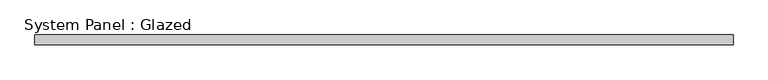
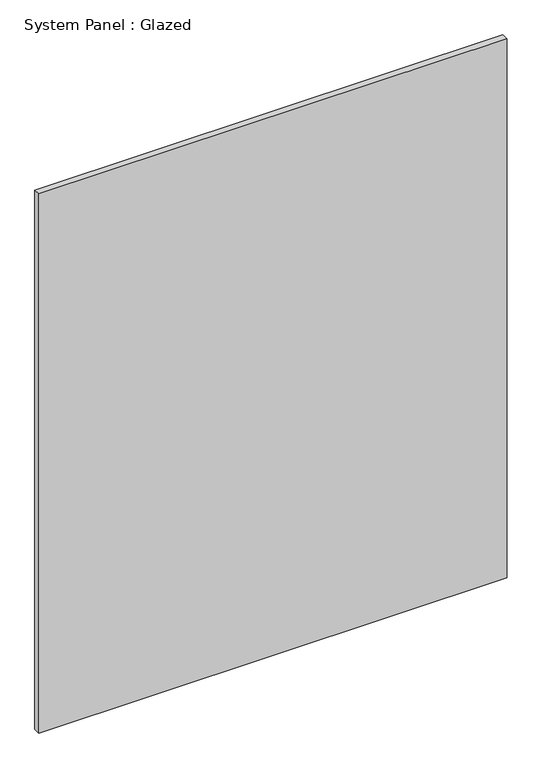
"""IFC4 building model written with IfcOpenShell, lengths in millimetres: plate geometry, System Panel : Glazed."""

from ifc_helpers import new_model, si_unit, origin, origin_with_axes, place, context, project, spatial, polyline, outline, extrude, source, transform, mapped, element, save


def system_panel_glazed_c41bd5e5(model_context):
    return source(origin(), model_context, "Body", "SweptSolid", [
        extrude(outline(polyline([(883.5, -49.5), (-883.5, -49.5), (-883.5, -24.5), (883.5, -24.5), (883.5, -49.5)])), origin_with_axes(), (0.0, 0.0, 1.0), 2150.0),
    ])


if __name__ == "__main__":
    model = new_model("IFC4")
    model_context = context("Model", 3, world=origin())
    ifc_project = project(units=[si_unit("LENGTHUNIT", "METRE", prefix="MILLI")], contexts=[model_context])
    site = spatial("IfcSite", under=ifc_project)
    building = spatial("IfcBuilding", under=site)
    placement = place(None, origin())
    system_panel_glazed_shape = system_panel_glazed_c41bd5e5(model_context)
    element("IfcPlate", 1, ObjectType="System Panel : Glazed", at=placement, inside=building, context=model_context, shape_type="MappedRepresentation", body=[
        mapped(system_panel_glazed_shape, transform((0.0, 0.0, 0.0), x_axis=(1.0, 0.0, 0.0), y_axis=(0.0, 1.0, 0.0), z_axis=(0.0, 0.0, 1.0))),
    ])
    save(model, "model.ifc")

# Revit data of these elements
# Type "System Panel : Glazed"
#   Keynote = "H11"
#   Construction Type Id = "GSP4R"
#   Analytic Construction = "1/8 in Pilkington single glazing"
#   Visual Light Transmittance = 0.9
#   Solar Heat Gain Coefficient = 0.86
#   Heat Transfer Coefficient (U) = 6.7069 W/(m²·K)
# Element 1 (IfcPlate, "System Panel : Glazed")
#   Materials on its faces: "Glass"
# Materials
#   "Glass": class "Glass", colour RGB 0 128 192, transparency 0.9, Description = "Soda Lime Glass", Cost = 0
